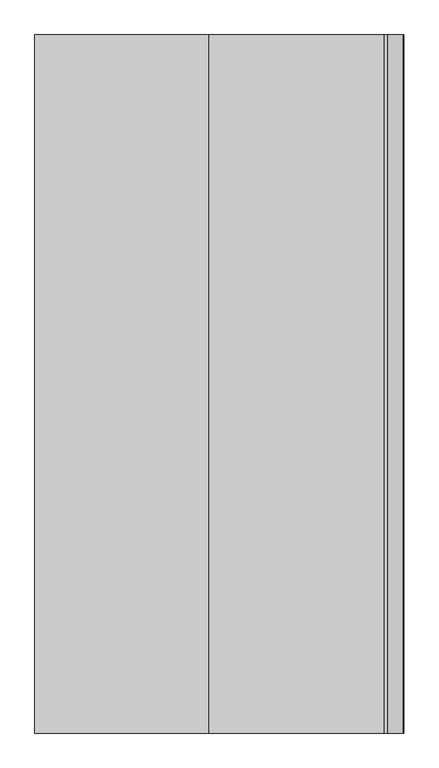
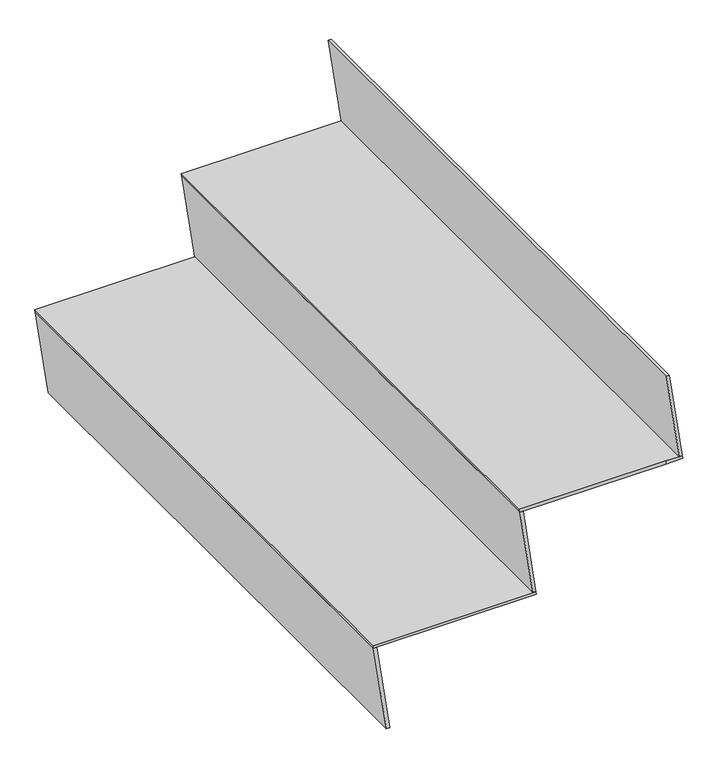
"""IFC4 building model written with IfcOpenShell, lengths in millimetres: stair flight geometry."""

from ifc_helpers import new_model, si_unit, origin, place, context, project, spatial, faceted_brep, source, transform, mapped, element, save


def stair_flight_c604de22(model_context):
    return source(origin(), model_context, "Body", "Brep", [
        faceted_brep([(15443.6343631, -17847.4618478, 173.9130435), (15444.4968631, -17847.4618478, 167.9130435), (15444.4968631, -16747.4618478, 167.9130435), (15443.6343631, -16747.4618478, 173.9130435), (15137.5726879, -16747.4618478, 173.9130435), (15137.5726879, -17847.4618478, 173.9130435), (15138.4351879, -17847.4618478, 167.9130435), (15138.4351879, -16747.4618478, 167.9130435)], [[[0, 1, 2, 3]], [[3, 4, 5, 0]], [[2, 1, 6, 7]], [[4, 3, 2, 7]], [[0, 5, 6, 1]], [[5, 4, 7, 6]]]),
        faceted_brep([(15138.4351879, -17847.4618478, 167.9130435), (15162.5726879, -17847.4618478, 0.0), (15168.6343631, -17847.4618478, 0.0), (15144.4968631, -17847.4618478, 167.9130435), (15138.4351879, -16747.4618478, 167.9130435), (15144.4968631, -16747.4618478, 167.9130435), (15168.6343631, -16747.4618478, 0.0), (15162.5726879, -16747.4618478, 0.0)], [[[0, 1, 2, 3]], [[4, 5, 6, 7]], [[1, 0, 4, 7]], [[2, 1, 7, 6]], [[3, 2, 6, 5]], [[0, 3, 5, 4]]]),
        faceted_brep([(15413.4351879, -17847.4618478, 341.826087), (15437.5726879, -17847.4618478, 173.9130435), (15443.6343631, -17847.4618478, 173.9130435), (15419.4968631, -17847.4618478, 341.826087), (15413.4351879, -16747.4618478, 341.826087), (15419.4968631, -16747.4618478, 341.826087), (15443.6343631, -16747.4618478, 173.9130435), (15437.5726879, -16747.4618478, 173.9130435)], [[[0, 1, 2, 3]], [[4, 5, 6, 7]], [[1, 0, 4, 7]], [[2, 1, 7, 6]], [[3, 2, 6, 5]], [[0, 3, 5, 4]]]),
        faceted_brep([(15688.4351879, -17847.4618478, 515.7391304), (15712.5726879, -17847.4618478, 347.826087), (15718.6343631, -17847.4618478, 347.826087), (15694.4968631, -17847.4618478, 515.7391304), (15688.4351879, -16747.4618478, 515.7391304), (15694.4968631, -16747.4618478, 515.7391304), (15718.6343631, -16747.4618478, 347.826087), (15712.5726879, -16747.4618478, 347.826087)], [[[0, 1, 2, 3]], [[4, 5, 6, 7]], [[1, 0, 4, 7]], [[2, 1, 7, 6]], [[3, 2, 6, 5]], [[0, 3, 5, 4]]]),
        faceted_brep([(15718.6343631, -16747.4618478, 347.826087), (15687.5726879, -16747.4618478, 347.826087), (15412.5726879, -16747.4618478, 347.826087), (15412.5726879, -17847.4618478, 347.826087), (15687.5726879, -17847.4618478, 347.826087), (15718.6343631, -17847.4618478, 347.826087), (15719.4968631, -16747.4618478, 341.826087), (15719.4968631, -17847.4618478, 341.826087), (15687.5726879, -17847.4618478, 341.826087), (15413.4351879, -17847.4618478, 341.826087), (15413.4351879, -16747.4618478, 341.826087), (15687.5726879, -16747.4618478, 341.826087)], [[[0, 1, 2, 3, 4, 5]], [[6, 7, 8, 9, 10, 11]], [[1, 0, 6, 11]], [[4, 3, 9, 8]], [[5, 7, 6, 0]], [[3, 2, 10, 9]], [[2, 1, 11, 10]], [[5, 4, 8, 7]]]),
    ])


if __name__ == "__main__":
    model = new_model("IFC4")
    model_context = context("Model", 3, world=origin())
    ifc_project = project(units=[si_unit("LENGTHUNIT", "METRE", prefix="MILLI")], contexts=[model_context])
    site = spatial("IfcSite", under=ifc_project)
    building = spatial("IfcBuilding", under=site)
    placement = place(None, origin())
    stair_flight_shape = stair_flight_c604de22(model_context)
    element("IfcStairFlight", 1, at=placement, inside=building, context=model_context, shape_type="MappedRepresentation", body=[
        mapped(stair_flight_shape, transform((0.0, 0.0, 0.0), x_axis=(1.0, 0.0, 0.0), y_axis=(0.0, 1.0, 0.0), z_axis=(0.0, 0.0, 1.0))),
    ])
    save(model, "model.ifc")

# Revit data of these elements
# Element 1 (IfcStairFlight)
#   Materials on its faces: "Acero, acabado de pintura, gris oscuro"
# Materials
#   "Acero, acabado de pintura, gris oscuro": class "Metal", colour RGB 89 89 89, transparency 0, Description = "Acero, acabado de pintura, gris oscuro, brillante", Cost = 0
